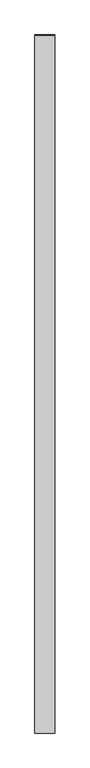
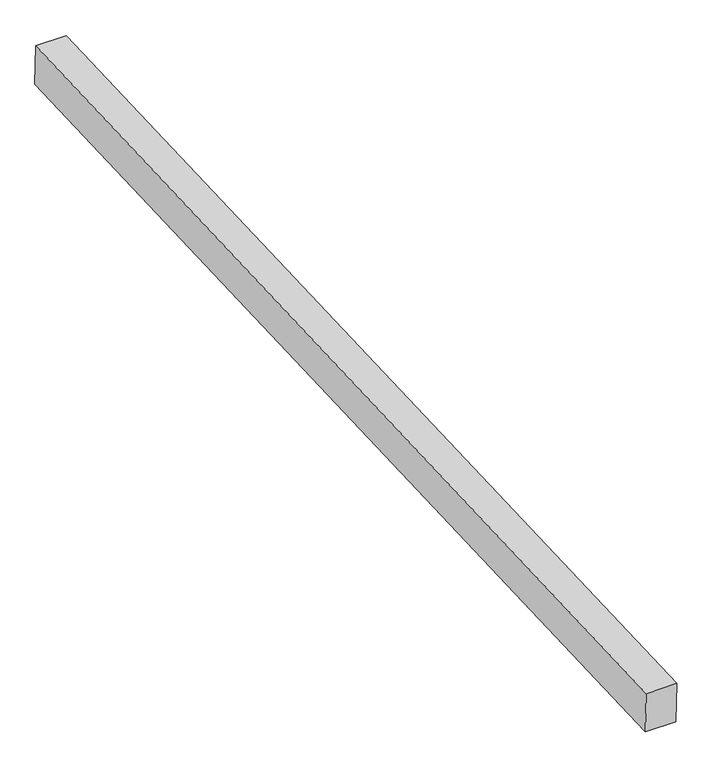
"""IFC4 building model written with IfcOpenShell, lengths in millimetres: proxy geometry, Generic Models 7:Generic Models 1:8:Generic Models 1:8 : Generic Models 7:Generic Models 1:337419:41 : Generic Models 7:Generic Models 1:8:Generic Models 1:8 : Generic Models 7:Generic Models 1:337419:315935."""

from ifc_helpers import new_model, si_unit, frame, origin, place, context, project, spatial, polyline, outline, extrude, source, transform, mapped, element, save


def generic_models_7672c0f3(model_context):
    return source(origin(), model_context, "Body", "SweptSolid", [
        extrude(outline(polyline([(-581229.2495411, 3818.908703), (-576356.3266468, 4021.9471569), (-576348.7597251, 3831.5971524), (-581221.3189223, 3628.5738526), (-581229.2495411, 3818.908703)])), frame((667198.0617239, 0.0, 0.0), z_axis=(1.0, 0.0, 0.0), x_axis=(0.0, 1.0, 0.0)), (0.0, 0.0, 1.0), 139.7),
    ])


if __name__ == "__main__":
    model = new_model("IFC4")
    model_context = context("Model", 3, world=origin())
    ifc_project = project(units=[si_unit("LENGTHUNIT", "METRE", prefix="MILLI")], contexts=[model_context])
    site = spatial("IfcSite", under=ifc_project)
    building = spatial("IfcBuilding", under=site)
    placement = place(None, origin())
    generic_models_shape = generic_models_7672c0f3(model_context)
    element("IfcBuildingElementProxy", 1, Name="Generic Models 7:Generic Models 1:8:Generic Models 1:8 : Generic Models 7:Generic Models 1:337419:41 : Generic Models 7:Generic Models 1:8:Generic Models 1:8 : Generic Models 7:Generic Models 1:337419:315935", ObjectType="Generic Models 7:Generic Models 1:8:Generic Models 1:8 : Generic Models 7:Generic Models 1:337419:41 : Generic Models 7:Generic Models 1:8:Generic Models 1:8 : Generic Models 7:Generic Models 1:337419:315935", at=placement, inside=building, context=model_context, shape_type="MappedRepresentation", body=[
        mapped(generic_models_shape, transform((0.0, 0.0, 0.0), x_axis=(1.0, 0.0, 0.0), y_axis=(0.0, 1.0, 0.0), z_axis=(0.0, 0.0, 1.0))),
    ])
    save(model, "model.ifc")

# Revit data of these elements
# Type "Generic Models 7:Generic Models 1:8:Generic Models 1:8 : Generic Models 7:Generic Models 1:337419:41 : Generic Models 7:Generic Models 1:8:Generic Models 1:8 : Generic Models 7:Generic Models 1:337419:315935"
#   NameOverride = "Generic Models 7:Generic Models 1:8:Generic Models 1:8 : Generic Models 7:Generic Models 1:337419:315935"
#   ObjectTypeOverride = "Generic Models 1:8 : Generic Models 7:Generic Models 1:337419"
#   Reference = "Generic Models 1"
#   Tag = "315935"
# Element 1 (IfcBuildingElementProxy, "Generic Models 7:Generic Models 1:8:Generic Models 1:8 : Generic Models 7:Generic Models 1:337419:41 : Generic Models 7:Generic Models 1:8:Generic Models 1:8 : Generic Models 7:Generic Models 1:337419:315935")
#   Materials on its faces: "5 1/2\" X 7 1/2\" EXTERIOR GRADE GLULAM BEAMS"
# Materials
#   "5 1/2\" X 7 1/2\" EXTERIOR GRADE GLULAM BEAMS": class "Wood", colour RGB 183 134 68, transparency 0, Keynote = "M06181300.01", Description = "Pinus Echinata", Cost = 0
